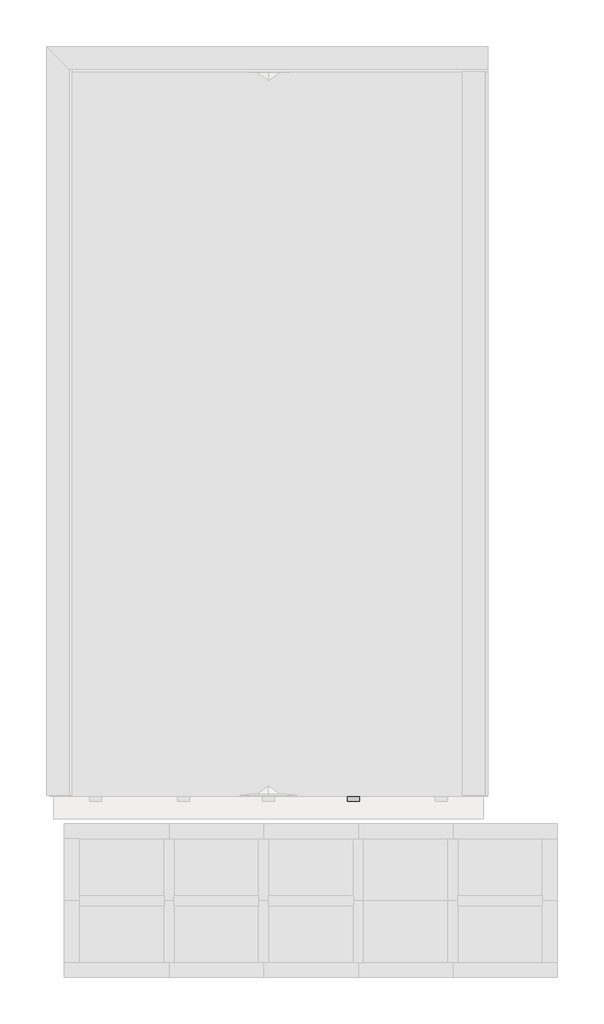
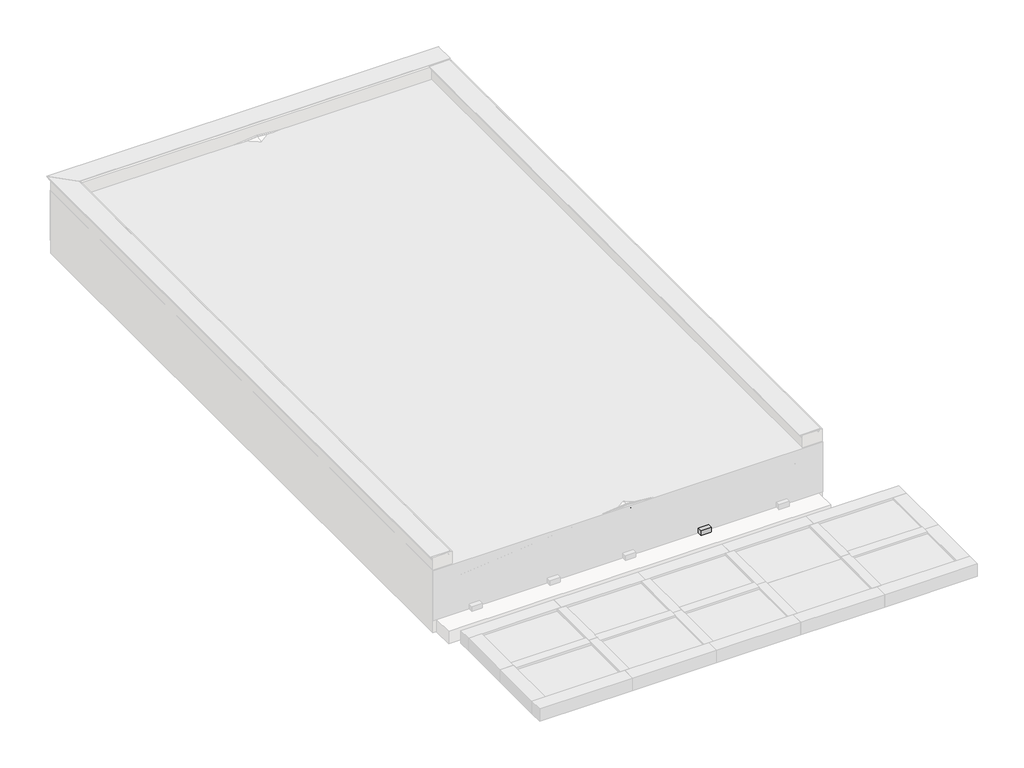
# One storey, part 2 of 3: 37 beams, 6 columns.
"""IFC4 building model written with IfcOpenShell, lengths in millimetres."""

import ifcopenshell
import ifcopenshell.guid

model = None  # the IFC model being written
_history = None  # IfcOwnerHistory: only IFC2X3 demands one
_inside = {}  # id of a spatial element -> (the spatial element, [elements in it])
_under = {}  # id of a project, library or spatial element -> (it, [spatial elements below it])
_declared = {}  # id of a project -> (the project, [libraries it declares])
_typed = {}  # id of a type object -> (the type object, [elements of that type])
_made_of = {}  # id of a material, layer set ... -> (it, [elements and type objects made of it])


def new_model(schema):
    """Start an empty IFC model of exactly this schema.

    Asked for "IFC4X3", IfcOpenShell would pick the latest addendum, in which some entities
    have other attributes; the version numbers below select the first issue.
    IFC2X3 requires an IfcOwnerHistory on every rooted entity: one is made here for all.
    """
    global model, _history
    if schema == "IFC4X3":
        model = ifcopenshell.file(schema_version=(4, 3, 0, 0))
    else:
        model = ifcopenshell.file(schema=schema)
    _inside.clear()
    _under.clear()
    _declared.clear()
    _typed.clear()
    _made_of.clear()
    _history = None
    if model.schema == "IFC2X3":
        org = make("IfcOrganization", Name="unknown")
        user = make(
            "IfcPersonAndOrganization",
            ThePerson=make("IfcPerson", FamilyName="unknown"),
            TheOrganization=org,
        )
        app = make(
            "IfcApplication",
            ApplicationDeveloper=org,
            Version="unknown",
            ApplicationFullName="unknown",
            ApplicationIdentifier="unknown",
        )
        _history = make(
            "IfcOwnerHistory",
            OwningUser=user,
            OwningApplication=app,
            ChangeAction="ADDED",
            CreationDate=0,
        )
    return model


def make(cls, **values):
    """One entity of the class cls with the attributes given. An attribute that is None is left unset."""
    return model.create_entity(
        cls, **{name: value for name, value in values.items() if value is not None}
    )


def rooted(cls, **values):
    """An entity with a GlobalId (a new one), such as an element, a storey or a relation."""
    return make(cls, GlobalId=ifcopenshell.guid.new(), OwnerHistory=_history, **values)


def si_unit(unit_type, name, prefix=None):
    """IfcSIUnit, for example si_unit("LENGTHUNIT", "METRE", prefix="MILLI")."""
    return make("IfcSIUnit", UnitType=unit_type, Prefix=prefix, Name=name)


def assignment(units):
    """IfcUnitAssignment: the units of a project."""
    return None if units is None else make("IfcUnitAssignment", Units=units)


def point(xyz):
    """IfcCartesianPoint."""
    return None if xyz is None else make("IfcCartesianPoint", Coordinates=xyz)


def direction(xyz):
    """IfcDirection."""
    return None if xyz is None else make("IfcDirection", DirectionRatios=xyz)


def frame(location, z_axis=None, x_axis=None):
    """IfcAxis2Placement3D, a coordinate frame: its origin and axes. An axis left out is left unset."""
    return make(
        "IfcAxis2Placement3D",
        Location=point(location),
        Axis=direction(z_axis),
        RefDirection=direction(x_axis),
    )


def frame_2d(location, x_axis=None):
    """IfcAxis2Placement2D, a coordinate frame in the plane: its origin and x axis."""
    return make(
        "IfcAxis2Placement2D", Location=point(location), RefDirection=direction(x_axis)
    )


def origin():
    """The frame at (0, 0, 0) with its axes left unset."""
    return frame((0.0, 0.0, 0.0))


def place(relative_to, where):
    """IfcLocalPlacement: puts the frame where relative to a parent placement (None: the world)."""
    return make(
        "IfcLocalPlacement", PlacementRelTo=relative_to, RelativePlacement=where
    )


def context(
    kind, dimensions, precision=None, world=None, true_north=None, identifier=None
):
    """IfcGeometricRepresentationContext, for example the 3D "Model" context."""
    return make(
        "IfcGeometricRepresentationContext",
        ContextIdentifier=identifier,
        ContextType=kind,
        CoordinateSpaceDimension=dimensions,
        Precision=precision,
        WorldCoordinateSystem=world,
        TrueNorth=true_north,
    )


def project(units=None, contexts=None):
    """IfcProject with its units and contexts."""
    return rooted(
        "IfcProject",
        Name="project",
        RepresentationContexts=contexts,
        UnitsInContext=assignment(units),
    )


def spatial(cls, under=None, at=None, **own):
    """A site, building, storey or space (cls), placed at a placement, below another one or the project."""
    s = rooted(cls, ObjectPlacement=at, **own)
    if under is not None:
        _under.setdefault(under.id(), (under, []))[1].append(s)
    return s


def polyline(points):
    """IfcPolyline through the points."""
    return make("IfcPolyline", Points=[point(p) for p in points])


def circle_curve(where, radius):
    """IfcCircle in the frame where."""
    return make("IfcCircle", Position=where, Radius=radius)


def trimmed(basis, trim1, trim2, sense, master):
    """IfcTrimmedCurve: the piece of a basis curve between two trims."""
    return make(
        "IfcTrimmedCurve",
        BasisCurve=basis,
        Trim1=trim1,
        Trim2=trim2,
        SenseAgreement=sense,
        MasterRepresentation=master,
    )


def segment(curve, same_sense, transition):
    """IfcCompositeCurveSegment."""
    return make(
        "IfcCompositeCurveSegment",
        Transition=transition,
        SameSense=same_sense,
        ParentCurve=curve,
    )


def composite_curve(segments, self_intersect=None):
    """IfcCompositeCurve: segments joined end to end."""
    return make("IfcCompositeCurve", Segments=segments, SelfIntersect=self_intersect)


def outline(outer, holes=None, kind="AREA"):
    """IfcArbitraryClosedProfileDef: a profile drawn as a closed curve; with holes, ...WithVoids."""
    if holes is None:
        return make("IfcArbitraryClosedProfileDef", ProfileType=kind, OuterCurve=outer)
    return make(
        "IfcArbitraryProfileDefWithVoids",
        ProfileType=kind,
        OuterCurve=outer,
        InnerCurves=holes,
    )


def extrude(swept, where, along, depth):
    """IfcExtrudedAreaSolid: the profile swept, set in the frame where, extruded along a direction by depth."""
    return make(
        "IfcExtrudedAreaSolid",
        SweptArea=swept,
        Position=where,
        ExtrudedDirection=direction(along),
        Depth=depth,
    )


def shape(context_of_items, identifier, shape_type, items):
    """IfcShapeRepresentation: the items that make up one representation, for example the "Body"."""
    return make(
        "IfcShapeRepresentation",
        ContextOfItems=context_of_items,
        RepresentationIdentifier=identifier,
        RepresentationType=shape_type,
        Items=items,
    )


def source(mapping_origin, context_of_items, identifier, shape_type, items):
    """IfcRepresentationMap: a shape defined once, which mapped items show again and again."""
    return make(
        "IfcRepresentationMap",
        MappingOrigin=mapping_origin,
        MappedRepresentation=shape(context_of_items, identifier, shape_type, items),
    )


def transform(
    local_origin,
    x_axis=None,
    y_axis=None,
    z_axis=None,
    scale=None,
    scale2=None,
    scale3=None,
    uniform=True,
):
    """IfcCartesianTransformationOperator3D, or its non-uniform kind. x_axis, y_axis, z_axis: its Axis1, 2, 3."""
    if uniform:
        return make(
            "IfcCartesianTransformationOperator3D",
            Axis1=direction(x_axis),
            Axis2=direction(y_axis),
            LocalOrigin=point(local_origin),
            Scale=scale,
            Axis3=direction(z_axis),
        )
    return make(
        "IfcCartesianTransformationOperator3DnonUniform",
        Axis1=direction(x_axis),
        Axis2=direction(y_axis),
        LocalOrigin=point(local_origin),
        Scale=scale,
        Axis3=direction(z_axis),
        Scale2=scale2,
        Scale3=scale3,
    )


def mapped(mapping_source, mapping_target):
    """IfcMappedItem: shows the shape of a source again, moved by a transform."""
    return make(
        "IfcMappedItem", MappingSource=mapping_source, MappingTarget=mapping_target
    )


def made_of(thing, what):
    """Note that an element or type object is made of a material, layer set ...; save() writes the relation."""
    if what is not None:
        _made_of.setdefault(what.id(), (what, []))[1].append(thing)
    return thing


def element(
    cls,
    number,
    at=None,
    inside=None,
    cuts=None,
    type_object=None,
    material=None,
    context=None,
    identifier="Body",
    shape_type=None,
    held_by="IfcProductDefinitionShape",
    body=None,
    shapes=None,
    **own,
):
    """One element of the class cls, such as IfcWall. Its Tag is "e" and its number.

    at: its placement. inside: the storey or other place that contains it. cuts: it is an
    opening in that element (IfcRelVoidsElement). A single representation is given by context,
    identifier, shape_type and body (its items); several are given by shapes. held_by: the class
    of the entity that holds the representations. save() writes the other relations.
    """
    e = rooted(cls, Tag="e%d" % number, ObjectPlacement=at, **own)
    if body is not None:
        shapes = [shape(context, identifier, shape_type, body)]
    if shapes is not None:
        e.Representation = make(held_by, Representations=shapes)
    if inside is not None:
        _inside.setdefault(inside.id(), (inside, []))[1].append(e)
    if cuts is not None:
        rooted(
            "IfcRelVoidsElement", RelatingBuildingElement=cuts, RelatedOpeningElement=e
        )
    if type_object is not None:
        _typed.setdefault(type_object.id(), (type_object, []))[1].append(e)
    return made_of(e, material)


def aggregate(whole, parts):
    """IfcRelAggregates: a whole, such as a stair, and the parts it consists of."""
    return rooted("IfcRelAggregates", RelatingObject=whole, RelatedObjects=parts)


def save(model, path):
    """Write the relations noted so far, then the file.

    IfcRelAggregates (storeys below a building ...), IfcRelContainedInSpatialStructure (elements
    in a storey), IfcRelDefinesByType, IfcRelAssociatesMaterial and IfcRelDeclares: one each for
    every whole, place, type object, material and project.
    """
    for whole, parts in _under.values():
        aggregate(whole, parts)
    for where, things in _inside.values():
        rooted(
            "IfcRelContainedInSpatialStructure",
            RelatedElements=things,
            RelatingStructure=where,
        )
    for kind, things in _typed.values():
        rooted("IfcRelDefinesByType", RelatedObjects=things, RelatingType=kind)
    for what, things in _made_of.values():
        rooted("IfcRelAssociatesMaterial", RelatedObjects=things, RelatingMaterial=what)
    for by, libraries in _declared.values():
        rooted("IfcRelDeclares", RelatingContext=by, RelatedDefinitions=libraries)
    model.write(path)


def cumeeira_telha_ondulada_fibrocimento_28917381(model_context):
    return source(origin(), model_context, "Body", "SweptSolid", [
        extrude(outline(composite_curve([segment(polyline([(58.3970135, 42.4437972), (53.9055884, 40.2467307)]), True, "CONTINUOUS"), segment(trimmed(circle_curve(frame_2d((-1.6029865, 13.0936483)), 61.7939461), [point((53.9055884, 40.2467307))], [point((-57.1115615, 40.2467307))], True, "CARTESIAN"), True, "CONTINUOUS"), segment(polyline([(-57.1115615, 40.2467307), (-61.6029865, 42.4437972)]), True, "CONTINUOUS"), segment(trimmed(circle_curve(frame_2d((-1.6029865, 13.0936483)), 66.7939461), [point((-61.6029865, 42.4437972))], [point((58.3970135, 42.4437972))], False, "CARTESIAN"), True, "CONTINUOUS")], self_intersect=False)), frame((-3626.5, 0.0, 0.0), z_axis=(1.0, 0.0, 0.0), x_axis=(0.0, 1.0, 0.0)), (0.0, 0.0, 1.0), 7253.0),
    ])


def viga_cumeeira_6x16cm_d80f05ee(model_context):
    return source(origin(), model_context, "Body", "SweptSolid", [
        extrude(outline(polyline([(3626.5, 30.0), (3626.5, -30.0), (-3626.5, -30.0), (-3626.5, 30.0), (3626.5, 30.0)])), frame((0.0, 0.0, -80.0), z_axis=(0.0, 0.0, 1.0), x_axis=(1.0, 0.0, 0.0)), (0.0, 0.0, 1.0), 160.0),
    ])


def column_1cffec27(model_context):
    return source(origin(), model_context, "Body", "SweptSolid", [
        extrude(outline(polyline([(30.0, 80.0), (30.0, -80.0), (-30.0, -80.0), (-30.0, 80.0), (30.0, 80.0)])), frame((0.0, 0.0, 3110.0), z_axis=(0.0, 0.0, 1.0), x_axis=(1.0, 0.0, 0.0)), (0.0, 0.0, 1.0), 238.0),
    ])


def column_35730ad5(model_context):
    return source(origin(), model_context, "Body", "SweptSolid", [
        extrude(outline(polyline([(30.0, 80.0), (30.0, -80.0), (-30.0, -80.0), (-30.0, 80.0), (30.0, 80.0)])), frame((0.0, 0.0, 3110.0), z_axis=(0.0, 0.0, 1.0), x_axis=(1.0, 0.0, 0.0)), (0.0, 0.0, 1.0), 197.9),
    ])


def column_00c463e4(model_context):
    return source(origin(), model_context, "Body", "SweptSolid", [
        extrude(outline(polyline([(30.0, 80.0), (30.0, -80.0), (-30.0, -80.0), (-30.0, 80.0), (30.0, 80.0)])), frame((0.0, 0.0, 3110.0), z_axis=(0.0, 0.0, 1.0), x_axis=(1.0, 0.0, 0.0)), (0.0, 0.0, 1.0), 109.8),
    ])


model = new_model("IFC4")

# Units and contexts
model_context = context("Model", 3, world=origin())
ifc_project = project(units=[si_unit("LENGTHUNIT", "METRE", prefix="MILLI")], contexts=[model_context])

# Site, building, storey
site = spatial("IfcSite", under=ifc_project)
building = spatial("IfcBuilding", under=site)
storey = spatial("IfcBuildingStorey", under=building, Name="COB. GARAGEM", Elevation=3050.0)

# Beams
placement = place(None, origin())
element("IfcBeam", 1, ObjectType="Madeira de lei : Berço 6x12cm", at=placement, inside=storey, context=model_context, shape_type="SweptSolid", body=[
    extrude(outline(polyline([(-9620.281307, 4423.9300153), (-9500.281307, 4423.9300153), (-9500.281307, 2423.9300153), (-9620.281307, 2423.9300153), (-9620.281307, 4423.9300153)])), frame((0.0, 0.0, 3050.0), z_axis=(0.0, 0.0, 1.0), x_axis=(1.0, 0.0, 0.0)), (0.0, 0.0, 1.0), 60.0),
])
element("IfcBeam", 2, ObjectType="Madeira de lei : Berço 6x12cm", at=placement, inside=storey, context=model_context, shape_type="SweptSolid", body=[
    extrude(outline(polyline([(-9620.281307, 2423.9300153), (-9500.281307, 2423.9300153), (-9500.281307, 423.9300153), (-9620.281307, 423.9300153), (-9620.281307, 2423.9300153)])), frame((0.0, 0.0, 3050.0), z_axis=(0.0, 0.0, 1.0), x_axis=(1.0, 0.0, 0.0)), (0.0, 0.0, 1.0), 60.0),
])
element("IfcBeam", 3, ObjectType="Madeira de lei : Berço 6x12cm", at=placement, inside=storey, context=model_context, shape_type="SweptSolid", body=[
    extrude(outline(polyline([(-8767.0824227, 4423.9300153), (-8647.0824227, 4423.9300153), (-8647.0824227, 2423.9300153), (-8767.0824227, 2423.9300153), (-8767.0824227, 4423.9300153)])), frame((0.0, 0.0, 3050.0), z_axis=(0.0, 0.0, 1.0), x_axis=(1.0, 0.0, 0.0)), (0.0, 0.0, 1.0), 60.0),
])
element("IfcBeam", 4, ObjectType="Madeira de lei : Berço 6x12cm", at=placement, inside=storey, context=model_context, shape_type="SweptSolid", body=[
    extrude(outline(polyline([(-8767.0824227, 2423.9300153), (-8647.0824227, 2423.9300153), (-8647.0824227, 423.9300153), (-8767.0824227, 423.9300153), (-8767.0824227, 2423.9300153)])), frame((0.0, 0.0, 3050.0), z_axis=(0.0, 0.0, 1.0), x_axis=(1.0, 0.0, 0.0)), (0.0, 0.0, 1.0), 60.0),
])
element("IfcBeam", 5, ObjectType="Madeira de lei : Berço 6x12cm", at=placement, inside=storey, context=model_context, shape_type="SweptSolid", body=[
    extrude(outline(polyline([(-8767.0824227, 423.9300153), (-8647.0824227, 423.9300153), (-8647.0824227, -236.0699847), (-8767.0824227, -236.0699847), (-8767.0824227, 423.9300153)])), frame((0.0, 0.0, 3050.0), z_axis=(0.0, 0.0, 1.0), x_axis=(1.0, 0.0, 0.0)), (0.0, 0.0, 1.0), 60.0),
])
element("IfcBeam", 6, ObjectType="Madeira de lei : Berço 6x12cm", at=placement, inside=storey, context=model_context, shape_type="SweptSolid", body=[
    extrude(outline(polyline([(-10473.4801913, 4423.9300153), (-10353.4801913, 4423.9300153), (-10353.4801913, 2423.9300153), (-10473.4801913, 2423.9300153), (-10473.4801913, 4423.9300153)])), frame((0.0, 0.0, 3050.0), z_axis=(0.0, 0.0, 1.0), x_axis=(1.0, 0.0, 0.0)), (0.0, 0.0, 1.0), 60.0),
])
element("IfcBeam", 7, ObjectType="Madeira de lei : Berço 6x12cm", at=placement, inside=storey, context=model_context, shape_type="SweptSolid", body=[
    extrude(outline(polyline([(-11356.5301913, 4423.9300153), (-11236.5301913, 4423.9300153), (-11236.5301913, 2423.9300153), (-11356.5301913, 2423.9300153), (-11356.5301913, 4423.9300153)])), frame((0.0, 0.0, 3050.0), z_axis=(0.0, 0.0, 1.0), x_axis=(1.0, 0.0, 0.0)), (0.0, 0.0, 1.0), 60.0),
])
cumeeira_telha_ondulada_fibrocimento_shape = cumeeira_telha_ondulada_fibrocimento_28917381(model_context)
element("IfcBeam", 8, ObjectType="Cumeeira Telha Ondulada : Fibrocimento", at=placement, inside=storey, context=model_context, shape_type="MappedRepresentation", body=[
    mapped(cumeeira_telha_ondulada_fibrocimento_shape, transform((-9560.281307, 3455.9300153, 3545.9751229), x_axis=(0.0, -1.0, 0.0), y_axis=(1.0, 0.0, 0.0), z_axis=(0.0, 0.0, 1.0))),
])
element("IfcBeam", 9, ObjectType="Telha Ondulada : Fibrocimento", at=placement, inside=storey, context=model_context, shape_type="SweptSolid", body=[
    extrude(outline(composite_curve([segment(trimmed(circle_curve(frame_2d((-58.7002979, -53.2060538)), 66.7939461), [point((-29.350149, 6.7939462))], [point((-29.350149, -113.2060538))], False, "CARTESIAN"), True, "CONTINUOUS"), segment(polyline([(-29.350149, -113.2060538), (-31.5472155, -108.7146288)]), True, "CONTINUOUS"), segment(trimmed(circle_curve(frame_2d((-58.7002979, -53.2060538)), 61.7939461), [point((-31.5472155, -108.7146288))], [point((-31.5472155, 2.3025211))], True, "CARTESIAN"), True, "CONTINUOUS"), segment(trimmed(circle_curve(frame_2d((0.0, 66.7939462)), 71.7939461), [point((-31.5472155, 2.3025211))], [point((-31.5472155, 131.2853712))], False, "CARTESIAN"), True, "CONTINUOUS"), segment(polyline([(-31.5472155, 131.2853712), (-29.350149, 126.7939462)]), True, "CONTINUOUS"), segment(trimmed(circle_curve(frame_2d((0.0, 66.7939462)), 66.7939461), [point((-29.350149, 126.7939462))], [point((-29.350149, 6.7939462))], True, "CARTESIAN"), True, "CONTINUOUS")], self_intersect=False)), frame((-11446.918865, 2229.326948, 3394.3067746), z_axis=(0.9950371902099892, 0.0, 0.09950371902099919), x_axis=(-0.09950371902099919, 0.0, 0.9950371902099892)), (0.0, 0.0, 1.0), 1886.8678854),
])
element("IfcBeam", 10, ObjectType="Telha Ondulada : Fibrocimento", at=placement, inside=storey, context=model_context, shape_type="SweptSolid", body=[
    extrude(outline(composite_curve([segment(trimmed(circle_curve(frame_2d((-58.7002979, -53.2060538)), 66.7939461), [point((-29.350149, 6.7939462))], [point((-29.350149, -113.2060538))], False, "CARTESIAN"), True, "CONTINUOUS"), segment(polyline([(-29.350149, -113.2060538), (-31.5472155, -108.7146288)]), True, "CONTINUOUS"), segment(trimmed(circle_curve(frame_2d((-58.7002979, -53.2060538)), 61.7939461), [point((-31.5472155, -108.7146288))], [point((-31.5472155, 2.3025211))], True, "CARTESIAN"), True, "CONTINUOUS"), segment(trimmed(circle_curve(frame_2d((0.0, 66.7939462)), 71.7939461), [point((-31.5472155, 2.3025211))], [point((-31.5472155, 131.2853712))], False, "CARTESIAN"), True, "CONTINUOUS"), segment(polyline([(-31.5472155, 131.2853712), (-29.350149, 126.7939462)]), True, "CONTINUOUS"), segment(trimmed(circle_curve(frame_2d((0.0, 66.7939462)), 66.7939461), [point((-29.350149, 126.7939462))], [point((-29.350149, 6.7939462))], True, "CARTESIAN"), True, "CONTINUOUS")], self_intersect=False)), frame((-11446.918865, 2473.826948, 3394.3067746), z_axis=(0.9950371902099892, 0.0, 0.09950371902099932), x_axis=(-0.09950371902099932, 0.0, 0.9950371902099892)), (0.0, 0.0, 1.0), 1886.8678854),
])
element("IfcBeam", 11, ObjectType="Telha Ondulada : Fibrocimento", at=placement, inside=storey, context=model_context, shape_type="SweptSolid", body=[
    extrude(outline(composite_curve([segment(trimmed(circle_curve(frame_2d((-58.7002979, -53.2060538)), 66.7939461), [point((-29.350149, 6.7939462))], [point((-29.350149, -113.2060538))], False, "CARTESIAN"), True, "CONTINUOUS"), segment(polyline([(-29.350149, -113.2060538), (-31.5472155, -108.7146288)]), True, "CONTINUOUS"), segment(trimmed(circle_curve(frame_2d((-58.7002979, -53.2060538)), 61.7939461), [point((-31.5472155, -108.7146288))], [point((-31.5472155, 2.3025211))], True, "CARTESIAN"), True, "CONTINUOUS"), segment(trimmed(circle_curve(frame_2d((0.0, 66.7939462)), 71.7939461), [point((-31.5472155, 2.3025211))], [point((-31.5472155, 131.2853712))], False, "CARTESIAN"), True, "CONTINUOUS"), segment(polyline([(-31.5472155, 131.2853712), (-29.350149, 126.7939462)]), True, "CONTINUOUS"), segment(trimmed(circle_curve(frame_2d((0.0, 66.7939462)), 66.7939461), [point((-29.350149, 126.7939462))], [point((-29.350149, 6.7939462))], True, "CARTESIAN"), True, "CONTINUOUS")], self_intersect=False)), frame((-11446.918865, 2718.326948, 3394.3067746), z_axis=(0.9950371902099892, 0.0, 0.09950371902099937), x_axis=(-0.09950371902099937, 0.0, 0.9950371902099892)), (0.0, 0.0, 1.0), 1886.8678854),
])
element("IfcBeam", 12, ObjectType="Telha Ondulada : Fibrocimento", at=placement, inside=storey, context=model_context, shape_type="SweptSolid", body=[
    extrude(outline(composite_curve([segment(trimmed(circle_curve(frame_2d((-58.7002979, -53.2060538)), 66.7939461), [point((-29.350149, 6.7939462))], [point((-29.350149, -113.2060538))], False, "CARTESIAN"), True, "CONTINUOUS"), segment(polyline([(-29.350149, -113.2060538), (-31.5472155, -108.7146288)]), True, "CONTINUOUS"), segment(trimmed(circle_curve(frame_2d((-58.7002979, -53.2060538)), 61.7939461), [point((-31.5472155, -108.7146288))], [point((-31.5472155, 2.3025211))], True, "CARTESIAN"), True, "CONTINUOUS"), segment(trimmed(circle_curve(frame_2d((0.0, 66.7939462)), 71.7939461), [point((-31.5472155, 2.3025211))], [point((-31.5472155, 131.2853712))], False, "CARTESIAN"), True, "CONTINUOUS"), segment(polyline([(-31.5472155, 131.2853712), (-29.350149, 126.7939462)]), True, "CONTINUOUS"), segment(trimmed(circle_curve(frame_2d((0.0, 66.7939462)), 66.7939461), [point((-29.350149, 126.7939462))], [point((-29.350149, 6.7939462))], True, "CARTESIAN"), True, "CONTINUOUS")], self_intersect=False)), frame((-11446.918865, 2962.826948, 3394.3067746), z_axis=(0.9950371902099892, 0.0, 0.09950371902099943), x_axis=(-0.09950371902099943, 0.0, 0.9950371902099892)), (0.0, 0.0, 1.0), 1886.8678854),
])
element("IfcBeam", 13, ObjectType="Telha Ondulada : Fibrocimento", at=placement, inside=storey, context=model_context, shape_type="SweptSolid", body=[
    extrude(outline(composite_curve([segment(trimmed(circle_curve(frame_2d((-58.7002979, -53.2060538)), 66.7939461), [point((-29.350149, 6.7939462))], [point((-29.350149, -113.2060538))], False, "CARTESIAN"), True, "CONTINUOUS"), segment(polyline([(-29.350149, -113.2060538), (-31.5472155, -108.7146288)]), True, "CONTINUOUS"), segment(trimmed(circle_curve(frame_2d((-58.7002979, -53.2060538)), 61.7939461), [point((-31.5472155, -108.7146288))], [point((-31.5472155, 2.3025211))], True, "CARTESIAN"), True, "CONTINUOUS"), segment(trimmed(circle_curve(frame_2d((0.0, 66.7939462)), 71.7939461), [point((-31.5472155, 2.3025211))], [point((-31.5472155, 131.2853712))], False, "CARTESIAN"), True, "CONTINUOUS"), segment(polyline([(-31.5472155, 131.2853712), (-29.350149, 126.7939462)]), True, "CONTINUOUS"), segment(trimmed(circle_curve(frame_2d((0.0, 66.7939462)), 66.7939461), [point((-29.350149, 126.7939462))], [point((-29.350149, 6.7939462))], True, "CARTESIAN"), True, "CONTINUOUS")], self_intersect=False)), frame((-11446.918865, 3207.326948, 3394.3067746), z_axis=(0.9950371902099892, 0.0, 0.09950371902099954), x_axis=(-0.09950371902099954, 0.0, 0.9950371902099892)), (0.0, 0.0, 1.0), 1886.8678854),
])
element("IfcBeam", 14, ObjectType="Telha Ondulada : Fibrocimento", at=placement, inside=storey, context=model_context, shape_type="SweptSolid", body=[
    extrude(outline(composite_curve([segment(trimmed(circle_curve(frame_2d((-58.7002979, -53.2060538)), 66.7939461), [point((-29.350149, 6.7939462))], [point((-29.350149, -113.2060538))], False, "CARTESIAN"), True, "CONTINUOUS"), segment(polyline([(-29.350149, -113.2060538), (-31.5472155, -108.7146288)]), True, "CONTINUOUS"), segment(trimmed(circle_curve(frame_2d((-58.7002979, -53.2060538)), 61.7939461), [point((-31.5472155, -108.7146288))], [point((-31.5472155, 2.3025211))], True, "CARTESIAN"), True, "CONTINUOUS"), segment(trimmed(circle_curve(frame_2d((0.0, 66.7939462)), 71.7939461), [point((-31.5472155, 2.3025211))], [point((-31.5472155, 131.2853712))], False, "CARTESIAN"), True, "CONTINUOUS"), segment(polyline([(-31.5472155, 131.2853712), (-29.350149, 126.7939462)]), True, "CONTINUOUS"), segment(trimmed(circle_curve(frame_2d((0.0, 66.7939462)), 66.7939461), [point((-29.350149, 126.7939462))], [point((-29.350149, 6.7939462))], True, "CARTESIAN"), True, "CONTINUOUS")], self_intersect=False)), frame((-11446.918865, 3451.826948, 3394.3067746), z_axis=(0.9950371902099892, 0.0, 0.09950371902099937), x_axis=(-0.09950371902099937, 0.0, 0.9950371902099892)), (0.0, 0.0, 1.0), 1886.8678854),
])
element("IfcBeam", 15, ObjectType="Telha Ondulada : Fibrocimento", at=placement, inside=storey, context=model_context, shape_type="SweptSolid", body=[
    extrude(outline(composite_curve([segment(trimmed(circle_curve(frame_2d((-58.7002979, -53.2060538)), 66.7939461), [point((-29.350149, 6.7939462))], [point((-29.350149, -113.2060538))], False, "CARTESIAN"), True, "CONTINUOUS"), segment(polyline([(-29.350149, -113.2060538), (-31.5472155, -108.7146288)]), True, "CONTINUOUS"), segment(trimmed(circle_curve(frame_2d((-58.7002979, -53.2060538)), 61.7939461), [point((-31.5472155, -108.7146288))], [point((-31.5472155, 2.3025211))], True, "CARTESIAN"), True, "CONTINUOUS"), segment(trimmed(circle_curve(frame_2d((0.0, 66.7939462)), 71.7939461), [point((-31.5472155, 2.3025211))], [point((-31.5472155, 131.2853712))], False, "CARTESIAN"), True, "CONTINUOUS"), segment(polyline([(-31.5472155, 131.2853712), (-29.350149, 126.7939462)]), True, "CONTINUOUS"), segment(trimmed(circle_curve(frame_2d((0.0, 66.7939462)), 66.7939461), [point((-29.350149, 126.7939462))], [point((-29.350149, 6.7939462))], True, "CARTESIAN"), True, "CONTINUOUS")], self_intersect=False)), frame((-11446.918865, 3696.326948, 3394.3067746), z_axis=(0.9950371902099892, 0.0, 0.09950371902099914), x_axis=(-0.09950371902099914, 0.0, 0.9950371902099892)), (0.0, 0.0, 1.0), 1886.8678854),
])
element("IfcBeam", 16, ObjectType="Telha Ondulada : Fibrocimento", at=placement, inside=storey, context=model_context, shape_type="SweptSolid", body=[
    extrude(outline(composite_curve([segment(trimmed(circle_curve(frame_2d((-58.7002979, -53.2060538)), 66.7939461), [point((-29.350149, 6.7939462))], [point((-29.350149, -113.2060538))], False, "CARTESIAN"), True, "CONTINUOUS"), segment(polyline([(-29.350149, -113.2060538), (-31.5472155, -108.7146288)]), True, "CONTINUOUS"), segment(trimmed(circle_curve(frame_2d((-58.7002979, -53.2060538)), 61.7939461), [point((-31.5472155, -108.7146288))], [point((-31.5472155, 2.3025211))], True, "CARTESIAN"), True, "CONTINUOUS"), segment(trimmed(circle_curve(frame_2d((0.0, 66.7939462)), 71.7939461), [point((-31.5472155, 2.3025211))], [point((-31.5472155, 131.2853712))], False, "CARTESIAN"), True, "CONTINUOUS"), segment(polyline([(-31.5472155, 131.2853712), (-29.350149, 126.7939462)]), True, "CONTINUOUS"), segment(trimmed(circle_curve(frame_2d((0.0, 66.7939462)), 66.7939461), [point((-29.350149, 126.7939462))], [point((-29.350149, 6.7939462))], True, "CARTESIAN"), True, "CONTINUOUS")], self_intersect=False)), frame((-11446.918865, 3940.826948, 3394.3067746), z_axis=(0.9950371902099892, 0.0, 0.09950371902099948), x_axis=(-0.09950371902099948, 0.0, 0.9950371902099892)), (0.0, 0.0, 1.0), 1886.8678854),
])
element("IfcBeam", 17, ObjectType="Telha Ondulada : Fibrocimento", at=placement, inside=storey, context=model_context, shape_type="SweptSolid", body=[
    extrude(outline(composite_curve([segment(trimmed(circle_curve(frame_2d((-58.7002979, -53.2060538)), 66.7939461), [point((-29.350149, 6.7939462))], [point((-29.350149, -113.2060538))], False, "CARTESIAN"), True, "CONTINUOUS"), segment(polyline([(-29.350149, -113.2060538), (-31.5472155, -108.7146288)]), True, "CONTINUOUS"), segment(trimmed(circle_curve(frame_2d((-58.7002979, -53.2060538)), 61.7939461), [point((-31.5472155, -108.7146288))], [point((-31.5472155, 2.3025211))], True, "CARTESIAN"), True, "CONTINUOUS"), segment(trimmed(circle_curve(frame_2d((0.0, 66.7939462)), 71.7939461), [point((-31.5472155, 2.3025211))], [point((-31.5472155, 131.2853712))], False, "CARTESIAN"), True, "CONTINUOUS"), segment(polyline([(-31.5472155, 131.2853712), (-29.350149, 126.7939462)]), True, "CONTINUOUS"), segment(trimmed(circle_curve(frame_2d((0.0, 66.7939462)), 66.7939461), [point((-29.350149, 126.7939462))], [point((-29.350149, 6.7939462))], True, "CARTESIAN"), True, "CONTINUOUS")], self_intersect=False)), frame((-11446.918865, 4185.326948, 3394.3067746), z_axis=(0.9950371902099892, 0.0, 0.09950371902099932), x_axis=(-0.09950371902099932, 0.0, 0.9950371902099892)), (0.0, 0.0, 1.0), 1886.8678854),
])
element("IfcBeam", 18, ObjectType="Telha Ondulada : Fibrocimento", at=placement, inside=storey, context=model_context, shape_type="SweptSolid", body=[
    extrude(outline(composite_curve([segment(trimmed(circle_curve(frame_2d((-58.7002979, -53.2060538)), 66.7939461), [point((-29.350149, 6.7939462))], [point((-29.350149, -113.2060538))], False, "CARTESIAN"), True, "CONTINUOUS"), segment(polyline([(-29.350149, -113.2060538), (-31.5472155, -108.7146288)]), True, "CONTINUOUS"), segment(trimmed(circle_curve(frame_2d((-58.7002979, -53.2060538)), 61.7939461), [point((-31.5472155, -108.7146288))], [point((-31.5472155, 2.3025211))], True, "CARTESIAN"), True, "CONTINUOUS"), segment(trimmed(circle_curve(frame_2d((0.0, 66.7939462)), 71.7939461), [point((-31.5472155, 2.3025211))], [point((-31.5472155, 131.2853712))], False, "CARTESIAN"), True, "CONTINUOUS"), segment(polyline([(-31.5472155, 131.2853712), (-29.350149, 126.7939462)]), True, "CONTINUOUS"), segment(trimmed(circle_curve(frame_2d((0.0, 66.7939462)), 66.7939461), [point((-29.350149, 126.7939462))], [point((-29.350149, 6.7939462))], True, "CARTESIAN"), True, "CONTINUOUS")], self_intersect=False)), frame((-11446.918865, 4429.826948, 3394.3067746), z_axis=(0.9950371902099892, 0.0, 0.09950371902099943), x_axis=(-0.09950371902099943, 0.0, 0.9950371902099892)), (0.0, 0.0, 1.0), 1886.8678854),
])
element("IfcBeam", 19, ObjectType="Telha Ondulada : Fibrocimento", at=placement, inside=storey, context=model_context, shape_type="SweptSolid", body=[
    extrude(outline(composite_curve([segment(trimmed(circle_curve(frame_2d((-58.7002979, -53.2060538)), 66.7939461), [point((-29.350149, 6.7939462))], [point((-29.350149, -113.2060538))], False, "CARTESIAN"), True, "CONTINUOUS"), segment(polyline([(-29.350149, -113.2060538), (-31.5472155, -108.7146288)]), True, "CONTINUOUS"), segment(trimmed(circle_curve(frame_2d((-58.7002979, -53.2060538)), 61.7939461), [point((-31.5472155, -108.7146288))], [point((-31.5472155, 2.3025211))], True, "CARTESIAN"), True, "CONTINUOUS"), segment(trimmed(circle_curve(frame_2d((0.0, 66.7939462)), 71.7939461), [point((-31.5472155, 2.3025211))], [point((-31.5472155, 131.2853712))], False, "CARTESIAN"), True, "CONTINUOUS"), segment(polyline([(-31.5472155, 131.2853712), (-29.350149, 126.7939462)]), True, "CONTINUOUS"), segment(trimmed(circle_curve(frame_2d((0.0, 66.7939462)), 66.7939461), [point((-29.350149, 126.7939462))], [point((-29.350149, 6.7939462))], True, "CARTESIAN"), True, "CONTINUOUS")], self_intersect=False)), frame((-11446.918865, 4674.326948, 3394.3067746), z_axis=(0.9950371902099892, 0.0, 0.09950371902099943), x_axis=(-0.09950371902099943, 0.0, 0.9950371902099892)), (0.0, 0.0, 1.0), 1886.8678854),
])
element("IfcBeam", 20, ObjectType="Telha Ondulada : Fibrocimento", at=placement, inside=storey, context=model_context, shape_type="SweptSolid", body=[
    extrude(outline(composite_curve([segment(trimmed(circle_curve(frame_2d((0.0, 66.7939462)), 66.7939461), [point((29.350149, 6.7939462))], [point((29.350149, 126.7939462))], True, "CARTESIAN"), True, "CONTINUOUS"), segment(polyline([(29.350149, 126.7939462), (31.5472155, 131.2853712)]), True, "CONTINUOUS"), segment(trimmed(circle_curve(frame_2d((0.0, 66.7939462)), 71.7939461), [point((31.5472155, 131.2853712))], [point((31.5472155, 2.3025211))], False, "CARTESIAN"), True, "CONTINUOUS"), segment(trimmed(circle_curve(frame_2d((58.7002979, -53.2060538)), 61.7939461), [point((31.5472155, 2.3025211))], [point((31.5472155, -108.7146288))], True, "CARTESIAN"), True, "CONTINUOUS"), segment(polyline([(31.5472155, -108.7146288), (29.350149, -113.2060538)]), True, "CONTINUOUS"), segment(trimmed(circle_curve(frame_2d((58.7002979, -53.2060538)), 66.7939461), [point((29.350149, -113.2060538))], [point((29.350149, 6.7939462))], False, "CARTESIAN"), True, "CONTINUOUS")], self_intersect=False)), frame((-7673.6437489, 28.826948, 3394.3067746), z_axis=(-0.9950371902099892, 0.0, 0.09950371902099979), x_axis=(-0.09950371902099979, 0.0, -0.9950371902099892)), (0.0, 0.0, 1.0), 1886.8678854),
])
element("IfcBeam", 21, ObjectType="Telha Ondulada : Fibrocimento", at=placement, inside=storey, context=model_context, shape_type="SweptSolid", body=[
    extrude(outline(composite_curve([segment(trimmed(circle_curve(frame_2d((0.0, 66.7939462)), 66.7939461), [point((29.350149, 6.7939462))], [point((29.350149, 126.7939462))], True, "CARTESIAN"), True, "CONTINUOUS"), segment(polyline([(29.350149, 126.7939462), (31.5472155, 131.2853712)]), True, "CONTINUOUS"), segment(trimmed(circle_curve(frame_2d((0.0, 66.7939462)), 71.7939461), [point((31.5472155, 131.2853712))], [point((31.5472155, 2.3025211))], False, "CARTESIAN"), True, "CONTINUOUS"), segment(trimmed(circle_curve(frame_2d((58.7002979, -53.2060538)), 61.7939461), [point((31.5472155, 2.3025211))], [point((31.5472155, -108.7146288))], True, "CARTESIAN"), True, "CONTINUOUS"), segment(polyline([(31.5472155, -108.7146288), (29.350149, -113.2060538)]), True, "CONTINUOUS"), segment(trimmed(circle_curve(frame_2d((58.7002979, -53.2060538)), 66.7939461), [point((29.350149, -113.2060538))], [point((29.350149, 6.7939462))], False, "CARTESIAN"), True, "CONTINUOUS")], self_intersect=False)), frame((-7673.6437489, 273.326948, 3394.3067746), z_axis=(-0.9950371902099892, 0.0, 0.09950371902099979), x_axis=(-0.09950371902099979, 0.0, -0.9950371902099892)), (0.0, 0.0, 1.0), 1886.8678854),
])
element("IfcBeam", 22, ObjectType="Telha Ondulada : Fibrocimento", at=placement, inside=storey, context=model_context, shape_type="SweptSolid", body=[
    extrude(outline(composite_curve([segment(trimmed(circle_curve(frame_2d((0.0, 66.7939462)), 66.7939461), [point((29.350149, 6.7939462))], [point((29.350149, 126.7939462))], True, "CARTESIAN"), True, "CONTINUOUS"), segment(polyline([(29.350149, 126.7939462), (31.5472155, 131.2853712)]), True, "CONTINUOUS"), segment(trimmed(circle_curve(frame_2d((0.0, 66.7939462)), 71.7939461), [point((31.5472155, 131.2853712))], [point((31.5472155, 2.3025211))], False, "CARTESIAN"), True, "CONTINUOUS"), segment(trimmed(circle_curve(frame_2d((58.7002979, -53.2060538)), 61.7939461), [point((31.5472155, 2.3025211))], [point((31.5472155, -108.7146288))], True, "CARTESIAN"), True, "CONTINUOUS"), segment(polyline([(31.5472155, -108.7146288), (29.350149, -113.2060538)]), True, "CONTINUOUS"), segment(trimmed(circle_curve(frame_2d((58.7002979, -53.2060538)), 66.7939461), [point((29.350149, -113.2060538))], [point((29.350149, 6.7939462))], False, "CARTESIAN"), True, "CONTINUOUS")], self_intersect=False)), frame((-7673.6437489, 517.826948, 3394.3067746), z_axis=(-0.9950371902099892, 0.0, 0.09950371902099979), x_axis=(-0.09950371902099979, 0.0, -0.9950371902099892)), (0.0, 0.0, 1.0), 1886.8678854),
])
element("IfcBeam", 23, ObjectType="Telha Ondulada : Fibrocimento", at=placement, inside=storey, context=model_context, shape_type="SweptSolid", body=[
    extrude(outline(composite_curve([segment(trimmed(circle_curve(frame_2d((0.0, 66.7939462)), 66.7939461), [point((29.350149, 6.7939462))], [point((29.350149, 126.7939462))], True, "CARTESIAN"), True, "CONTINUOUS"), segment(polyline([(29.350149, 126.7939462), (31.5472155, 131.2853712)]), True, "CONTINUOUS"), segment(trimmed(circle_curve(frame_2d((0.0, 66.7939462)), 71.7939461), [point((31.5472155, 131.2853712))], [point((31.5472155, 2.3025211))], False, "CARTESIAN"), True, "CONTINUOUS"), segment(trimmed(circle_curve(frame_2d((58.7002979, -53.2060538)), 61.7939461), [point((31.5472155, 2.3025211))], [point((31.5472155, -108.7146288))], True, "CARTESIAN"), True, "CONTINUOUS"), segment(polyline([(31.5472155, -108.7146288), (29.350149, -113.2060538)]), True, "CONTINUOUS"), segment(trimmed(circle_curve(frame_2d((58.7002979, -53.2060538)), 66.7939461), [point((29.350149, -113.2060538))], [point((29.350149, 6.7939462))], False, "CARTESIAN"), True, "CONTINUOUS")], self_intersect=False)), frame((-7673.6437489, 762.326948, 3394.3067746), z_axis=(-0.9950371902099892, 0.0, 0.09950371902099979), x_axis=(-0.09950371902099979, 0.0, -0.9950371902099892)), (0.0, 0.0, 1.0), 1886.8678854),
])
element("IfcBeam", 24, ObjectType="Telha Ondulada : Fibrocimento", at=placement, inside=storey, context=model_context, shape_type="SweptSolid", body=[
    extrude(outline(composite_curve([segment(trimmed(circle_curve(frame_2d((0.0, 66.7939462)), 66.7939461), [point((29.350149, 6.7939462))], [point((29.350149, 126.7939462))], True, "CARTESIAN"), True, "CONTINUOUS"), segment(polyline([(29.350149, 126.7939462), (31.5472155, 131.2853712)]), True, "CONTINUOUS"), segment(trimmed(circle_curve(frame_2d((0.0, 66.7939462)), 71.7939461), [point((31.5472155, 131.2853712))], [point((31.5472155, 2.3025211))], False, "CARTESIAN"), True, "CONTINUOUS"), segment(trimmed(circle_curve(frame_2d((58.7002979, -53.2060538)), 61.7939461), [point((31.5472155, 2.3025211))], [point((31.5472155, -108.7146288))], True, "CARTESIAN"), True, "CONTINUOUS"), segment(polyline([(31.5472155, -108.7146288), (29.350149, -113.2060538)]), True, "CONTINUOUS"), segment(trimmed(circle_curve(frame_2d((58.7002979, -53.2060538)), 66.7939461), [point((29.350149, -113.2060538))], [point((29.350149, 6.7939462))], False, "CARTESIAN"), True, "CONTINUOUS")], self_intersect=False)), frame((-7673.6437489, 1006.826948, 3394.3067746), z_axis=(-0.9950371902099892, 0.0, 0.09950371902099979), x_axis=(-0.09950371902099979, 0.0, -0.9950371902099892)), (0.0, 0.0, 1.0), 1886.8678854),
])
element("IfcBeam", 25, ObjectType="Telha Ondulada : Fibrocimento", at=placement, inside=storey, context=model_context, shape_type="SweptSolid", body=[
    extrude(outline(composite_curve([segment(trimmed(circle_curve(frame_2d((0.0, 66.7939462)), 66.7939461), [point((29.350149, 6.7939462))], [point((29.350149, 126.7939462))], True, "CARTESIAN"), True, "CONTINUOUS"), segment(polyline([(29.350149, 126.7939462), (31.5472155, 131.2853712)]), True, "CONTINUOUS"), segment(trimmed(circle_curve(frame_2d((0.0, 66.7939462)), 71.7939461), [point((31.5472155, 131.2853712))], [point((31.5472155, 2.3025211))], False, "CARTESIAN"), True, "CONTINUOUS"), segment(trimmed(circle_curve(frame_2d((58.7002979, -53.2060538)), 61.7939461), [point((31.5472155, 2.3025211))], [point((31.5472155, -108.7146288))], True, "CARTESIAN"), True, "CONTINUOUS"), segment(polyline([(31.5472155, -108.7146288), (29.350149, -113.2060538)]), True, "CONTINUOUS"), segment(trimmed(circle_curve(frame_2d((58.7002979, -53.2060538)), 66.7939461), [point((29.350149, -113.2060538))], [point((29.350149, 6.7939462))], False, "CARTESIAN"), True, "CONTINUOUS")], self_intersect=False)), frame((-7673.6437489, 1251.326948, 3394.3067746), z_axis=(-0.9950371902099892, 0.0, 0.09950371902099979), x_axis=(-0.09950371902099979, 0.0, -0.9950371902099892)), (0.0, 0.0, 1.0), 1886.8678854),
])
element("IfcBeam", 26, ObjectType="Telha Ondulada : Fibrocimento", at=placement, inside=storey, context=model_context, shape_type="SweptSolid", body=[
    extrude(outline(composite_curve([segment(trimmed(circle_curve(frame_2d((0.0, 66.7939462)), 66.7939461), [point((29.350149, 6.7939462))], [point((29.350149, 126.7939462))], True, "CARTESIAN"), True, "CONTINUOUS"), segment(polyline([(29.350149, 126.7939462), (31.5472155, 131.2853712)]), True, "CONTINUOUS"), segment(trimmed(circle_curve(frame_2d((0.0, 66.7939462)), 71.7939461), [point((31.5472155, 131.2853712))], [point((31.5472155, 2.3025211))], False, "CARTESIAN"), True, "CONTINUOUS"), segment(trimmed(circle_curve(frame_2d((58.7002979, -53.2060538)), 61.7939461), [point((31.5472155, 2.3025211))], [point((31.5472155, -108.7146288))], True, "CARTESIAN"), True, "CONTINUOUS"), segment(polyline([(31.5472155, -108.7146288), (29.350149, -113.2060538)]), True, "CONTINUOUS"), segment(trimmed(circle_curve(frame_2d((58.7002979, -53.2060538)), 66.7939461), [point((29.350149, -113.2060538))], [point((29.350149, 6.7939462))], False, "CARTESIAN"), True, "CONTINUOUS")], self_intersect=False)), frame((-7673.6437489, 1495.826948, 3394.3067746), z_axis=(-0.9950371902099892, 0.0, 0.09950371902099979), x_axis=(-0.09950371902099979, 0.0, -0.9950371902099892)), (0.0, 0.0, 1.0), 1886.8678854),
])
element("IfcBeam", 27, ObjectType="Telha Ondulada : Fibrocimento", at=placement, inside=storey, context=model_context, shape_type="SweptSolid", body=[
    extrude(outline(composite_curve([segment(trimmed(circle_curve(frame_2d((0.0, 66.7939462)), 66.7939461), [point((29.350149, 6.7939462))], [point((29.350149, 126.7939462))], True, "CARTESIAN"), True, "CONTINUOUS"), segment(polyline([(29.350149, 126.7939462), (31.5472155, 131.2853712)]), True, "CONTINUOUS"), segment(trimmed(circle_curve(frame_2d((0.0, 66.7939462)), 71.7939461), [point((31.5472155, 131.2853712))], [point((31.5472155, 2.3025211))], False, "CARTESIAN"), True, "CONTINUOUS"), segment(trimmed(circle_curve(frame_2d((58.7002979, -53.2060538)), 61.7939461), [point((31.5472155, 2.3025211))], [point((31.5472155, -108.7146288))], True, "CARTESIAN"), True, "CONTINUOUS"), segment(polyline([(31.5472155, -108.7146288), (29.350149, -113.2060538)]), True, "CONTINUOUS"), segment(trimmed(circle_curve(frame_2d((58.7002979, -53.2060538)), 66.7939461), [point((29.350149, -113.2060538))], [point((29.350149, 6.7939462))], False, "CARTESIAN"), True, "CONTINUOUS")], self_intersect=False)), frame((-7673.6437489, 1740.326948, 3394.3067746), z_axis=(-0.9950371902099892, 0.0, 0.09950371902099979), x_axis=(-0.09950371902099979, 0.0, -0.9950371902099892)), (0.0, 0.0, 1.0), 1886.8678854),
])
element("IfcBeam", 28, ObjectType="Telha Ondulada : Fibrocimento", at=placement, inside=storey, context=model_context, shape_type="SweptSolid", body=[
    extrude(outline(composite_curve([segment(trimmed(circle_curve(frame_2d((0.0, 66.7939462)), 66.7939461), [point((29.350149, 6.7939462))], [point((29.350149, 126.7939462))], True, "CARTESIAN"), True, "CONTINUOUS"), segment(polyline([(29.350149, 126.7939462), (31.5472155, 131.2853712)]), True, "CONTINUOUS"), segment(trimmed(circle_curve(frame_2d((0.0, 66.7939462)), 71.7939461), [point((31.5472155, 131.2853712))], [point((31.5472155, 2.3025211))], False, "CARTESIAN"), True, "CONTINUOUS"), segment(trimmed(circle_curve(frame_2d((58.7002979, -53.2060538)), 61.7939461), [point((31.5472155, 2.3025211))], [point((31.5472155, -108.7146288))], True, "CARTESIAN"), True, "CONTINUOUS"), segment(polyline([(31.5472155, -108.7146288), (29.350149, -113.2060538)]), True, "CONTINUOUS"), segment(trimmed(circle_curve(frame_2d((58.7002979, -53.2060538)), 66.7939461), [point((29.350149, -113.2060538))], [point((29.350149, 6.7939462))], False, "CARTESIAN"), True, "CONTINUOUS")], self_intersect=False)), frame((-7673.6437489, 1984.826948, 3394.3067746), z_axis=(-0.9950371902099892, 0.0, 0.09950371902099979), x_axis=(-0.09950371902099979, 0.0, -0.9950371902099892)), (0.0, 0.0, 1.0), 1886.8678854),
])
element("IfcBeam", 29, ObjectType="Telha Ondulada : Fibrocimento", at=placement, inside=storey, context=model_context, shape_type="SweptSolid", body=[
    extrude(outline(composite_curve([segment(trimmed(circle_curve(frame_2d((0.0, 66.7939462)), 66.7939461), [point((29.350149, 6.7939462))], [point((29.350149, 126.7939462))], True, "CARTESIAN"), True, "CONTINUOUS"), segment(polyline([(29.350149, 126.7939462), (31.5472155, 131.2853712)]), True, "CONTINUOUS"), segment(trimmed(circle_curve(frame_2d((0.0, 66.7939462)), 71.7939461), [point((31.5472155, 131.2853712))], [point((31.5472155, 2.3025211))], False, "CARTESIAN"), True, "CONTINUOUS"), segment(trimmed(circle_curve(frame_2d((58.7002979, -53.2060538)), 61.7939461), [point((31.5472155, 2.3025211))], [point((31.5472155, -108.7146288))], True, "CARTESIAN"), True, "CONTINUOUS"), segment(polyline([(31.5472155, -108.7146288), (29.350149, -113.2060538)]), True, "CONTINUOUS"), segment(trimmed(circle_curve(frame_2d((58.7002979, -53.2060538)), 66.7939461), [point((29.350149, -113.2060538))], [point((29.350149, 6.7939462))], False, "CARTESIAN"), True, "CONTINUOUS")], self_intersect=False)), frame((-7673.6437489, 2229.326948, 3394.3067746), z_axis=(-0.9950371902099892, 0.0, 0.09950371902099979), x_axis=(-0.09950371902099979, 0.0, -0.9950371902099892)), (0.0, 0.0, 1.0), 1886.8678854),
])
element("IfcBeam", 30, ObjectType="Telha Ondulada : Fibrocimento", at=placement, inside=storey, context=model_context, shape_type="SweptSolid", body=[
    extrude(outline(composite_curve([segment(trimmed(circle_curve(frame_2d((0.0, 66.7939462)), 66.7939461), [point((29.350149, 6.7939462))], [point((29.350149, 126.7939462))], True, "CARTESIAN"), True, "CONTINUOUS"), segment(polyline([(29.350149, 126.7939462), (31.5472155, 131.2853712)]), True, "CONTINUOUS"), segment(trimmed(circle_curve(frame_2d((0.0, 66.7939462)), 71.7939461), [point((31.5472155, 131.2853712))], [point((31.5472155, 2.3025211))], False, "CARTESIAN"), True, "CONTINUOUS"), segment(trimmed(circle_curve(frame_2d((58.7002979, -53.2060538)), 61.7939461), [point((31.5472155, 2.3025211))], [point((31.5472155, -108.7146288))], True, "CARTESIAN"), True, "CONTINUOUS"), segment(polyline([(31.5472155, -108.7146288), (29.350149, -113.2060538)]), True, "CONTINUOUS"), segment(trimmed(circle_curve(frame_2d((58.7002979, -53.2060538)), 66.7939461), [point((29.350149, -113.2060538))], [point((29.350149, 6.7939462))], False, "CARTESIAN"), True, "CONTINUOUS")], self_intersect=False)), frame((-7673.6437489, 2473.826948, 3394.3067746), z_axis=(-0.9950371902099892, 0.0, 0.09950371902099979), x_axis=(-0.09950371902099979, 0.0, -0.9950371902099892)), (0.0, 0.0, 1.0), 1886.8678854),
])
element("IfcBeam", 31, ObjectType="Telha Ondulada : Fibrocimento", at=placement, inside=storey, context=model_context, shape_type="SweptSolid", body=[
    extrude(outline(composite_curve([segment(trimmed(circle_curve(frame_2d((0.0, 66.7939462)), 66.7939461), [point((29.350149, 6.7939462))], [point((29.350149, 126.7939462))], True, "CARTESIAN"), True, "CONTINUOUS"), segment(polyline([(29.350149, 126.7939462), (31.5472155, 131.2853712)]), True, "CONTINUOUS"), segment(trimmed(circle_curve(frame_2d((0.0, 66.7939462)), 71.7939461), [point((31.5472155, 131.2853712))], [point((31.5472155, 2.3025211))], False, "CARTESIAN"), True, "CONTINUOUS"), segment(trimmed(circle_curve(frame_2d((58.7002979, -53.2060538)), 61.7939461), [point((31.5472155, 2.3025211))], [point((31.5472155, -108.7146288))], True, "CARTESIAN"), True, "CONTINUOUS"), segment(polyline([(31.5472155, -108.7146288), (29.350149, -113.2060538)]), True, "CONTINUOUS"), segment(trimmed(circle_curve(frame_2d((58.7002979, -53.2060538)), 66.7939461), [point((29.350149, -113.2060538))], [point((29.350149, 6.7939462))], False, "CARTESIAN"), True, "CONTINUOUS")], self_intersect=False)), frame((-7673.6437489, 2718.326948, 3394.3067746), z_axis=(-0.9950371902099892, 0.0, 0.09950371902099979), x_axis=(-0.09950371902099979, 0.0, -0.9950371902099892)), (0.0, 0.0, 1.0), 1886.8678854),
])
element("IfcBeam", 32, ObjectType="Telha Ondulada : Fibrocimento", at=placement, inside=storey, context=model_context, shape_type="SweptSolid", body=[
    extrude(outline(composite_curve([segment(trimmed(circle_curve(frame_2d((0.0, 66.7939462)), 66.7939461), [point((29.350149, 6.7939462))], [point((29.350149, 126.7939462))], True, "CARTESIAN"), True, "CONTINUOUS"), segment(polyline([(29.350149, 126.7939462), (31.5472155, 131.2853712)]), True, "CONTINUOUS"), segment(trimmed(circle_curve(frame_2d((0.0, 66.7939462)), 71.7939461), [point((31.5472155, 131.2853712))], [point((31.5472155, 2.3025211))], False, "CARTESIAN"), True, "CONTINUOUS"), segment(trimmed(circle_curve(frame_2d((58.7002979, -53.2060538)), 61.7939461), [point((31.5472155, 2.3025211))], [point((31.5472155, -108.7146288))], True, "CARTESIAN"), True, "CONTINUOUS"), segment(polyline([(31.5472155, -108.7146288), (29.350149, -113.2060538)]), True, "CONTINUOUS"), segment(trimmed(circle_curve(frame_2d((58.7002979, -53.2060538)), 66.7939461), [point((29.350149, -113.2060538))], [point((29.350149, 6.7939462))], False, "CARTESIAN"), True, "CONTINUOUS")], self_intersect=False)), frame((-7673.6437489, 2962.826948, 3394.3067746), z_axis=(-0.9950371902099892, 0.0, 0.09950371902099979), x_axis=(-0.09950371902099979, 0.0, -0.9950371902099892)), (0.0, 0.0, 1.0), 1886.8678854),
])
element("IfcBeam", 33, ObjectType="Telha Ondulada : Fibrocimento", at=placement, inside=storey, context=model_context, shape_type="SweptSolid", body=[
    extrude(outline(composite_curve([segment(trimmed(circle_curve(frame_2d((0.0, 66.7939462)), 66.7939461), [point((29.350149, 6.7939462))], [point((29.350149, 126.7939462))], True, "CARTESIAN"), True, "CONTINUOUS"), segment(polyline([(29.350149, 126.7939462), (31.5472155, 131.2853712)]), True, "CONTINUOUS"), segment(trimmed(circle_curve(frame_2d((0.0, 66.7939462)), 71.7939461), [point((31.5472155, 131.2853712))], [point((31.5472155, 2.3025211))], False, "CARTESIAN"), True, "CONTINUOUS"), segment(trimmed(circle_curve(frame_2d((58.7002979, -53.2060538)), 61.7939461), [point((31.5472155, 2.3025211))], [point((31.5472155, -108.7146288))], True, "CARTESIAN"), True, "CONTINUOUS"), segment(polyline([(31.5472155, -108.7146288), (29.350149, -113.2060538)]), True, "CONTINUOUS"), segment(trimmed(circle_curve(frame_2d((58.7002979, -53.2060538)), 66.7939461), [point((29.350149, -113.2060538))], [point((29.350149, 6.7939462))], False, "CARTESIAN"), True, "CONTINUOUS")], self_intersect=False)), frame((-7673.6437489, 3207.326948, 3394.3067746), z_axis=(-0.9950371902099892, 0.0, 0.09950371902099979), x_axis=(-0.09950371902099979, 0.0, -0.9950371902099892)), (0.0, 0.0, 1.0), 1886.8678854),
])
element("IfcBeam", 34, ObjectType="Telha Ondulada : Fibrocimento", at=placement, inside=storey, context=model_context, shape_type="SweptSolid", body=[
    extrude(outline(composite_curve([segment(trimmed(circle_curve(frame_2d((0.0, 66.7939462)), 66.7939461), [point((29.350149, 6.7939462))], [point((29.350149, 126.7939462))], True, "CARTESIAN"), True, "CONTINUOUS"), segment(polyline([(29.350149, 126.7939462), (31.5472155, 131.2853712)]), True, "CONTINUOUS"), segment(trimmed(circle_curve(frame_2d((0.0, 66.7939462)), 71.7939461), [point((31.5472155, 131.2853712))], [point((31.5472155, 2.3025211))], False, "CARTESIAN"), True, "CONTINUOUS"), segment(trimmed(circle_curve(frame_2d((58.7002979, -53.2060538)), 61.7939461), [point((31.5472155, 2.3025211))], [point((31.5472155, -108.7146288))], True, "CARTESIAN"), True, "CONTINUOUS"), segment(polyline([(31.5472155, -108.7146288), (29.350149, -113.2060538)]), True, "CONTINUOUS"), segment(trimmed(circle_curve(frame_2d((58.7002979, -53.2060538)), 66.7939461), [point((29.350149, -113.2060538))], [point((29.350149, 6.7939462))], False, "CARTESIAN"), True, "CONTINUOUS")], self_intersect=False)), frame((-7673.6437489, 3451.826948, 3394.3067746), z_axis=(-0.9950371902099892, 0.0, 0.09950371902099979), x_axis=(-0.09950371902099979, 0.0, -0.9950371902099892)), (0.0, 0.0, 1.0), 1886.8678854),
])
element("IfcBeam", 35, ObjectType="Telha Ondulada : Fibrocimento", at=placement, inside=storey, context=model_context, shape_type="SweptSolid", body=[
    extrude(outline(composite_curve([segment(trimmed(circle_curve(frame_2d((0.0, 66.7939462)), 66.7939461), [point((29.350149, 6.7939462))], [point((29.350149, 126.7939462))], True, "CARTESIAN"), True, "CONTINUOUS"), segment(polyline([(29.350149, 126.7939462), (31.5472155, 131.2853712)]), True, "CONTINUOUS"), segment(trimmed(circle_curve(frame_2d((0.0, 66.7939462)), 71.7939461), [point((31.5472155, 131.2853712))], [point((31.5472155, 2.3025211))], False, "CARTESIAN"), True, "CONTINUOUS"), segment(trimmed(circle_curve(frame_2d((58.7002979, -53.2060538)), 61.7939461), [point((31.5472155, 2.3025211))], [point((31.5472155, -108.7146288))], True, "CARTESIAN"), True, "CONTINUOUS"), segment(polyline([(31.5472155, -108.7146288), (29.350149, -113.2060538)]), True, "CONTINUOUS"), segment(trimmed(circle_curve(frame_2d((58.7002979, -53.2060538)), 66.7939461), [point((29.350149, -113.2060538))], [point((29.350149, 6.7939462))], False, "CARTESIAN"), True, "CONTINUOUS")], self_intersect=False)), frame((-7673.6437489, 3696.326948, 3394.3067746), z_axis=(-0.9950371902099892, 0.0, 0.09950371902099979), x_axis=(-0.09950371902099979, 0.0, -0.9950371902099892)), (0.0, 0.0, 1.0), 1886.8678854),
])
element("IfcBeam", 36, ObjectType="Telha Ondulada : Fibrocimento", at=placement, inside=storey, context=model_context, shape_type="SweptSolid", body=[
    extrude(outline(composite_curve([segment(trimmed(circle_curve(frame_2d((0.0, 66.7939462)), 66.7939461), [point((29.350149, 6.7939462))], [point((29.350149, 126.7939462))], True, "CARTESIAN"), True, "CONTINUOUS"), segment(polyline([(29.350149, 126.7939462), (31.5472155, 131.2853712)]), True, "CONTINUOUS"), segment(trimmed(circle_curve(frame_2d((0.0, 66.7939462)), 71.7939461), [point((31.5472155, 131.2853712))], [point((31.5472155, 2.3025211))], False, "CARTESIAN"), True, "CONTINUOUS"), segment(trimmed(circle_curve(frame_2d((58.7002979, -53.2060538)), 61.7939461), [point((31.5472155, 2.3025211))], [point((31.5472155, -108.7146288))], True, "CARTESIAN"), True, "CONTINUOUS"), segment(polyline([(31.5472155, -108.7146288), (29.350149, -113.2060538)]), True, "CONTINUOUS"), segment(trimmed(circle_curve(frame_2d((58.7002979, -53.2060538)), 66.7939461), [point((29.350149, -113.2060538))], [point((29.350149, 6.7939462))], False, "CARTESIAN"), True, "CONTINUOUS")], self_intersect=False)), frame((-7673.6437489, 3940.826948, 3394.3067746), z_axis=(-0.9950371902099892, 0.0, 0.09950371902099979), x_axis=(-0.09950371902099979, 0.0, -0.9950371902099892)), (0.0, 0.0, 1.0), 1886.8678854),
])
viga_cumeeira_6x16cm_shape = viga_cumeeira_6x16cm_d80f05ee(model_context)
element("IfcBeam", 37, ObjectType="Madeira de lei : Viga Cumeeira 6x16cm", at=placement, inside=storey, context=model_context, shape_type="MappedRepresentation", body=[
    mapped(viga_cumeeira_6x16cm_shape, transform((-9560.281307, 3455.9300153, 3427.8), x_axis=(0.0, -1.0, 0.0), y_axis=(1.0, 0.0, 0.0), z_axis=(0.0, 0.0, 1.0))),
])

# Columns
column_shape = column_1cffec27(model_context)
element("IfcColumn", 38, ObjectType="Madeira de lei-Coluna : Pontalete 6X16cm", at=placement, inside=storey, context=model_context, shape_type="MappedRepresentation", body=[
    mapped(column_shape, transform((-9560.281307, 3423.9300153, 0.0), x_axis=(1.0, 0.0, 0.0), y_axis=(0.0, 1.0, 0.0), z_axis=(0.0, 0.0, 1.0))),
])
element("IfcColumn", 39, ObjectType="Madeira de lei-Coluna : Pontalete 6X16cm", at=placement, inside=storey, context=model_context, shape_type="MappedRepresentation", body=[
    mapped(column_shape, transform((-9560.281307, 1423.9300153, 0.0), x_axis=(1.0, 0.0, 0.0), y_axis=(0.0, 1.0, 0.0), z_axis=(0.0, 0.0, 1.0))),
])
column_2_shape = column_35730ad5(model_context)
element("IfcColumn", 40, ObjectType="Madeira de lei-Coluna : Pontalete 6X16cm", at=placement, inside=storey, context=model_context, shape_type="MappedRepresentation", body=[
    mapped(column_2_shape, transform((-8707.0824227, 3423.9300153, 0.0), x_axis=(1.0, 0.0, 0.0), y_axis=(0.0, 1.0, 0.0), z_axis=(0.0, 0.0, 1.0))),
])
element("IfcColumn", 41, ObjectType="Madeira de lei-Coluna : Pontalete 6X16cm", at=placement, inside=storey, context=model_context, shape_type="MappedRepresentation", body=[
    mapped(column_2_shape, transform((-8707.0824227, 1423.9300153, 0.0), x_axis=(1.0, 0.0, 0.0), y_axis=(0.0, 1.0, 0.0), z_axis=(0.0, 0.0, 1.0))),
])
element("IfcColumn", 42, ObjectType="Madeira de lei-Coluna : Pontalete 6X16cm", at=placement, inside=storey, context=model_context, shape_type="MappedRepresentation", body=[
    mapped(column_2_shape, transform((-10413.4801913, 3423.9300153, 0.0), x_axis=(1.0, 0.0, 0.0), y_axis=(0.0, 1.0, 0.0), z_axis=(0.0, 0.0, 1.0))),
])
column_3_shape = column_00c463e4(model_context)
element("IfcColumn", 43, ObjectType="Madeira de lei-Coluna : Pontalete 6X16cm", at=placement, inside=storey, context=model_context, shape_type="MappedRepresentation", body=[
    mapped(column_3_shape, transform((-11296.5301913, 3423.9300153, 0.0), x_axis=(1.0, 0.0, 0.0), y_axis=(0.0, 1.0, 0.0), z_axis=(0.0, 0.0, 1.0))),
])

save(model, "model.ifc")

# Revit data of these elements
# Project information
#   Design Option = "Main Model"
#   Project Status = "Status do projeto"
#   Client Name = "JOÃO MATIAS SOARES"
#   Project Address = "RUA SÉRGIO DIAS, LOTE 30, QUADRA G, MONTE MINEIRO/MG"
#   Project Name = "CONSTRUÇÃO RESIDENCIA UNIFAMILIAR"
#   Project Number = "034/2017"
#   Zona = "ZER - 01"
#   CA Mín = "0.2"
#   CA Básico = "1"
#   CA Máx = "2"
#   TO Máx = "50"
#   Gabarito Máx = "10"
#   TP Mín = "15"
#   Área Total do Terreno = "620.00 m²"
#   Multifamiliar - Vagas Veículos/Pavto = "0"
#   Multifamiliar - Vagas Bicicletas/Pavto = "0"
#   Multifamiliar - % Vagas PNMR = "0"
#   Multifamiliar - % Vagas Motos = "0"
#   Outros - Área p/ 1 Veículo = "0.00 m²"
#   Outros - Área p/ 1 Bicicleta = "0.00 m²"
#   Outros - Área p/ 1 Utilitário = "0.00 m²"
#   Outros - % Vagas PNMR = "0"
#   Outros - % Vagas Motos = "0"
# Type "Madeira de lei : Berço 6x12cm"
#   A = 0.02 m²
#   Length [instance default] = 1.524 m
#   b = 0.06 m
#   d = 0.12 m
#   Structural Material [instance default] = none
#   Assembly Code = ""
# Type "Cumeeira Telha Ondulada : Fibrocimento"
#   Cost = 5
#   Length [instance default] = 1.524 m
#   b = 0.07 m
#   h = 0.16 m
#   Structural Material = .TELHA DE FIBROCIMENTO
#   Assembly Code = ""
# Type "Telha Ondulada : Fibrocimento"
#   Description = "TELHA ONDULADA FIBROCIMENTO"
#   Cost = 5
#   Length [instance default] = 1.524 m
#   b = 0.07 m
#   h = 0.16 m
#   Structural Material = .TELHA DE FIBROCIMENTO
#   Assembly Code = ""
# Type "Madeira de lei : Viga Cumeeira 6x16cm"
#   A = 0.02 m²
#   Length [instance default] = 1.524 m
#   b = 0.06 m
#   d = 0.16 m
#   Structural Material [instance default] = none
#   Assembly Code = ""
# Type "Madeira de lei-Coluna : Pontalete 6X16cm"
#   A = 0.01952 m²
#   b = 0.06 m
#   d = 0.16 m
#   Structural Material [instance default] = none
#   Assembly Code = ""
# Elements 1, 2, 3, 4, 6, 7 (IfcBeam, "Madeira de lei : Berço 6x12cm")
#   Comments = ""
#   Uso = "TELHADOS ESTRUTURAS"
#   Compr Cmcl = 6.00 m
#   Structural Material = .MADEIRAMENTO
